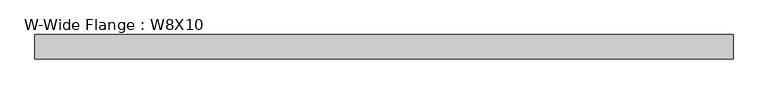
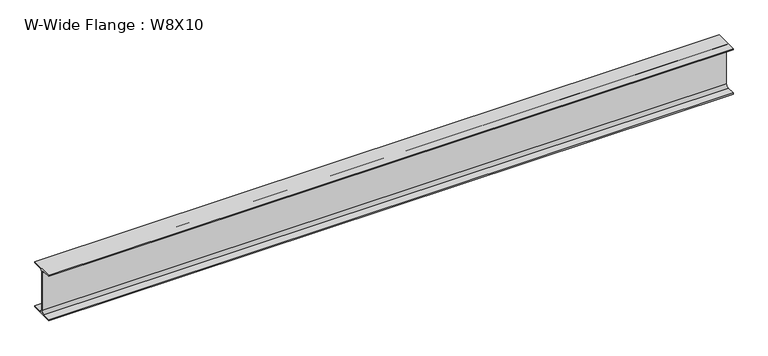
"""IFC4 building model written with IfcOpenShell, lengths in millimetres: beam geometry, W-Wide Flange : W8X10."""

import ifcopenshell
import ifcopenshell.guid

model = None  # the IFC model being written
_history = None  # IfcOwnerHistory: only IFC2X3 demands one
_inside = {}  # id of a spatial element -> (the spatial element, [elements in it])
_under = {}  # id of a project, library or spatial element -> (it, [spatial elements below it])
_declared = {}  # id of a project -> (the project, [libraries it declares])
_typed = {}  # id of a type object -> (the type object, [elements of that type])
_made_of = {}  # id of a material, layer set ... -> (it, [elements and type objects made of it])


def new_model(schema):
    """Start an empty IFC model of exactly this schema.

    Asked for "IFC4X3", IfcOpenShell would pick the latest addendum, in which some entities
    have other attributes; the version numbers below select the first issue.
    IFC2X3 requires an IfcOwnerHistory on every rooted entity: one is made here for all.
    """
    global model, _history
    if schema == "IFC4X3":
        model = ifcopenshell.file(schema_version=(4, 3, 0, 0))
    else:
        model = ifcopenshell.file(schema=schema)
    _inside.clear()
    _under.clear()
    _declared.clear()
    _typed.clear()
    _made_of.clear()
    _history = None
    if model.schema == "IFC2X3":
        org = make("IfcOrganization", Name="unknown")
        user = make(
            "IfcPersonAndOrganization",
            ThePerson=make("IfcPerson", FamilyName="unknown"),
            TheOrganization=org,
        )
        app = make(
            "IfcApplication",
            ApplicationDeveloper=org,
            Version="unknown",
            ApplicationFullName="unknown",
            ApplicationIdentifier="unknown",
        )
        _history = make(
            "IfcOwnerHistory",
            OwningUser=user,
            OwningApplication=app,
            ChangeAction="ADDED",
            CreationDate=0,
        )
    return model


def make(cls, **values):
    """One entity of the class cls with the attributes given. An attribute that is None is left unset."""
    return model.create_entity(
        cls, **{name: value for name, value in values.items() if value is not None}
    )


def rooted(cls, **values):
    """An entity with a GlobalId (a new one), such as an element, a storey or a relation."""
    return make(cls, GlobalId=ifcopenshell.guid.new(), OwnerHistory=_history, **values)


def si_unit(unit_type, name, prefix=None):
    """IfcSIUnit, for example si_unit("LENGTHUNIT", "METRE", prefix="MILLI")."""
    return make("IfcSIUnit", UnitType=unit_type, Prefix=prefix, Name=name)


def assignment(units):
    """IfcUnitAssignment: the units of a project."""
    return None if units is None else make("IfcUnitAssignment", Units=units)


def point(xyz):
    """IfcCartesianPoint."""
    return None if xyz is None else make("IfcCartesianPoint", Coordinates=xyz)


def direction(xyz):
    """IfcDirection."""
    return None if xyz is None else make("IfcDirection", DirectionRatios=xyz)


def frame(location, z_axis=None, x_axis=None):
    """IfcAxis2Placement3D, a coordinate frame: its origin and axes. An axis left out is left unset."""
    return make(
        "IfcAxis2Placement3D",
        Location=point(location),
        Axis=direction(z_axis),
        RefDirection=direction(x_axis),
    )


def frame_2d(location, x_axis=None):
    """IfcAxis2Placement2D, a coordinate frame in the plane: its origin and x axis."""
    return make(
        "IfcAxis2Placement2D", Location=point(location), RefDirection=direction(x_axis)
    )


def origin():
    """The frame at (0, 0, 0) with its axes left unset."""
    return frame((0.0, 0.0, 0.0))


def place(relative_to, where):
    """IfcLocalPlacement: puts the frame where relative to a parent placement (None: the world)."""
    return make(
        "IfcLocalPlacement", PlacementRelTo=relative_to, RelativePlacement=where
    )


def context(
    kind, dimensions, precision=None, world=None, true_north=None, identifier=None
):
    """IfcGeometricRepresentationContext, for example the 3D "Model" context."""
    return make(
        "IfcGeometricRepresentationContext",
        ContextIdentifier=identifier,
        ContextType=kind,
        CoordinateSpaceDimension=dimensions,
        Precision=precision,
        WorldCoordinateSystem=world,
        TrueNorth=true_north,
    )


def project(units=None, contexts=None):
    """IfcProject with its units and contexts."""
    return rooted(
        "IfcProject",
        Name="project",
        RepresentationContexts=contexts,
        UnitsInContext=assignment(units),
    )


def spatial(cls, under=None, at=None, **own):
    """A site, building, storey or space (cls), placed at a placement, below another one or the project."""
    s = rooted(cls, ObjectPlacement=at, **own)
    if under is not None:
        _under.setdefault(under.id(), (under, []))[1].append(s)
    return s


def polyline(points):
    """IfcPolyline through the points."""
    return make("IfcPolyline", Points=[point(p) for p in points])


def circle_curve(where, radius):
    """IfcCircle in the frame where."""
    return make("IfcCircle", Position=where, Radius=radius)


def trimmed(basis, trim1, trim2, sense, master):
    """IfcTrimmedCurve: the piece of a basis curve between two trims."""
    return make(
        "IfcTrimmedCurve",
        BasisCurve=basis,
        Trim1=trim1,
        Trim2=trim2,
        SenseAgreement=sense,
        MasterRepresentation=master,
    )


def segment(curve, same_sense, transition):
    """IfcCompositeCurveSegment."""
    return make(
        "IfcCompositeCurveSegment",
        Transition=transition,
        SameSense=same_sense,
        ParentCurve=curve,
    )


def composite_curve(segments, self_intersect=None):
    """IfcCompositeCurve: segments joined end to end."""
    return make("IfcCompositeCurve", Segments=segments, SelfIntersect=self_intersect)


def outline(outer, holes=None, kind="AREA"):
    """IfcArbitraryClosedProfileDef: a profile drawn as a closed curve; with holes, ...WithVoids."""
    if holes is None:
        return make("IfcArbitraryClosedProfileDef", ProfileType=kind, OuterCurve=outer)
    return make(
        "IfcArbitraryProfileDefWithVoids",
        ProfileType=kind,
        OuterCurve=outer,
        InnerCurves=holes,
    )


def extrude(swept, where, along, depth):
    """IfcExtrudedAreaSolid: the profile swept, set in the frame where, extruded along a direction by depth."""
    return make(
        "IfcExtrudedAreaSolid",
        SweptArea=swept,
        Position=where,
        ExtrudedDirection=direction(along),
        Depth=depth,
    )


def shape(context_of_items, identifier, shape_type, items):
    """IfcShapeRepresentation: the items that make up one representation, for example the "Body"."""
    return make(
        "IfcShapeRepresentation",
        ContextOfItems=context_of_items,
        RepresentationIdentifier=identifier,
        RepresentationType=shape_type,
        Items=items,
    )


def source(mapping_origin, context_of_items, identifier, shape_type, items):
    """IfcRepresentationMap: a shape defined once, which mapped items show again and again."""
    return make(
        "IfcRepresentationMap",
        MappingOrigin=mapping_origin,
        MappedRepresentation=shape(context_of_items, identifier, shape_type, items),
    )


def transform(
    local_origin,
    x_axis=None,
    y_axis=None,
    z_axis=None,
    scale=None,
    scale2=None,
    scale3=None,
    uniform=True,
):
    """IfcCartesianTransformationOperator3D, or its non-uniform kind. x_axis, y_axis, z_axis: its Axis1, 2, 3."""
    if uniform:
        return make(
            "IfcCartesianTransformationOperator3D",
            Axis1=direction(x_axis),
            Axis2=direction(y_axis),
            LocalOrigin=point(local_origin),
            Scale=scale,
            Axis3=direction(z_axis),
        )
    return make(
        "IfcCartesianTransformationOperator3DnonUniform",
        Axis1=direction(x_axis),
        Axis2=direction(y_axis),
        LocalOrigin=point(local_origin),
        Scale=scale,
        Axis3=direction(z_axis),
        Scale2=scale2,
        Scale3=scale3,
    )


def mapped(mapping_source, mapping_target):
    """IfcMappedItem: shows the shape of a source again, moved by a transform."""
    return make(
        "IfcMappedItem", MappingSource=mapping_source, MappingTarget=mapping_target
    )


def made_of(thing, what):
    """Note that an element or type object is made of a material, layer set ...; save() writes the relation."""
    if what is not None:
        _made_of.setdefault(what.id(), (what, []))[1].append(thing)
    return thing


def element(
    cls,
    number,
    at=None,
    inside=None,
    cuts=None,
    type_object=None,
    material=None,
    context=None,
    identifier="Body",
    shape_type=None,
    held_by="IfcProductDefinitionShape",
    body=None,
    shapes=None,
    **own,
):
    """One element of the class cls, such as IfcWall. Its Tag is "e" and its number.

    at: its placement. inside: the storey or other place that contains it. cuts: it is an
    opening in that element (IfcRelVoidsElement). A single representation is given by context,
    identifier, shape_type and body (its items); several are given by shapes. held_by: the class
    of the entity that holds the representations. save() writes the other relations.
    """
    e = rooted(cls, Tag="e%d" % number, ObjectPlacement=at, **own)
    if body is not None:
        shapes = [shape(context, identifier, shape_type, body)]
    if shapes is not None:
        e.Representation = make(held_by, Representations=shapes)
    if inside is not None:
        _inside.setdefault(inside.id(), (inside, []))[1].append(e)
    if cuts is not None:
        rooted(
            "IfcRelVoidsElement", RelatingBuildingElement=cuts, RelatedOpeningElement=e
        )
    if type_object is not None:
        _typed.setdefault(type_object.id(), (type_object, []))[1].append(e)
    return made_of(e, material)


def aggregate(whole, parts):
    """IfcRelAggregates: a whole, such as a stair, and the parts it consists of."""
    return rooted("IfcRelAggregates", RelatingObject=whole, RelatedObjects=parts)


def save(model, path):
    """Write the relations noted so far, then the file.

    IfcRelAggregates (storeys below a building ...), IfcRelContainedInSpatialStructure (elements
    in a storey), IfcRelDefinesByType, IfcRelAssociatesMaterial and IfcRelDeclares: one each for
    every whole, place, type object, material and project.
    """
    for whole, parts in _under.values():
        aggregate(whole, parts)
    for where, things in _inside.values():
        rooted(
            "IfcRelContainedInSpatialStructure",
            RelatedElements=things,
            RelatingStructure=where,
        )
    for kind, things in _typed.values():
        rooted("IfcRelDefinesByType", RelatedObjects=things, RelatingType=kind)
    for what, things in _made_of.values():
        rooted("IfcRelAssociatesMaterial", RelatedObjects=things, RelatingMaterial=what)
    for by, libraries in _declared.values():
        rooted("IfcRelDeclares", RelatingContext=by, RelatedDefinitions=libraries)
    model.write(path)


def w_wide_flange_w8x10_0a1c7429(model_context):
    return source(origin(), model_context, "Body", "SweptSolid", [
        extrude(outline(composite_curve([segment(polyline([(50.038, -94.996), (50.038, -100.203), (-50.038, -100.203), (-50.038, -94.996), (-14.4145, -94.996)]), True, "CONTINUOUS"), segment(trimmed(circle_curve(frame_2d((-14.4145, -82.7405)), 12.2555), [point((-14.4145, -94.996))], [point((-2.159, -82.7405))], True, "CARTESIAN"), True, "CONTINUOUS"), segment(polyline([(-2.159, -82.7405), (-2.159, 82.7405)]), True, "CONTINUOUS"), segment(trimmed(circle_curve(frame_2d((-14.4145, 82.7405)), 12.2555), [point((-2.159, 82.7405))], [point((-14.4145, 94.996))], True, "CARTESIAN"), True, "CONTINUOUS"), segment(polyline([(-14.4145, 94.996), (-50.038, 94.996), (-50.038, 100.203), (50.038, 100.203), (50.038, 94.996), (14.4145, 94.996)]), True, "CONTINUOUS"), segment(trimmed(circle_curve(frame_2d((14.4145, 82.7405)), 12.2555), [point((14.4145, 94.996))], [point((2.159, 82.7405))], True, "CARTESIAN"), True, "CONTINUOUS"), segment(polyline([(2.159, 82.7405), (2.159, -82.7405)]), True, "CONTINUOUS"), segment(trimmed(circle_curve(frame_2d((14.4145, -82.7405)), 12.2555), [point((2.159, -82.7405))], [point((14.4145, -94.996))], True, "CARTESIAN"), True, "CONTINUOUS"), segment(polyline([(14.4145, -94.996), (50.038, -94.996)]), True, "CONTINUOUS")], self_intersect=False)), frame((-1117.6, 0.0, 0.0), z_axis=(1.0, 0.0, 0.0), x_axis=(0.0, 1.0, 0.0)), (0.0, 0.0, 1.0), 2854.1219816),
    ])


if __name__ == "__main__":
    model = new_model("IFC4")
    model_context = context("Model", 3, world=origin())
    ifc_project = project(units=[si_unit("LENGTHUNIT", "METRE", prefix="MILLI")], contexts=[model_context])
    site = spatial("IfcSite", under=ifc_project)
    building = spatial("IfcBuilding", under=site)
    placement = place(None, origin())
    w_wide_flange_w8x10_shape = w_wide_flange_w8x10_0a1c7429(model_context)
    element("IfcBeam", 1, ObjectType="W-Wide Flange : W8X10", at=placement, inside=building, context=model_context, shape_type="MappedRepresentation", body=[
        mapped(w_wide_flange_w8x10_shape, transform((0.0, 0.0, 0.0), x_axis=(1.0, 0.0, 0.0), y_axis=(0.0, 1.0, 0.0), z_axis=(0.0, 0.0, 1.0))),
    ])
    save(model, "model.ifc")

# Revit data of these elements
# Type "W-Wide Flange : W8X10"
#   Assembly Code = "B10"
#   W = 10
#   Length [instance default] = 5' - 0"
#   bf = 0' - 3.94"
#   d = 0' - 7.89"
#   k = 0' - 0 11/16"
#   k2 = 0' - 0.4825"
#   tf = 0' - 0.205"
#   tw = 0' - 0.17"
#   A = 0.0205556 SF
#   Structural Material [instance default] = Steel ASTM A992
# Element 1 (IfcBeam, "W-Wide Flange : W8X10")
#   Structural Material = none
# Materials
#   "Steel ASTM A992": class "Metal", colour RGB 189 187 185, transparency 0, Description = "Structural steel 50ksi", Cost = 0
